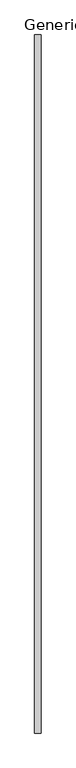
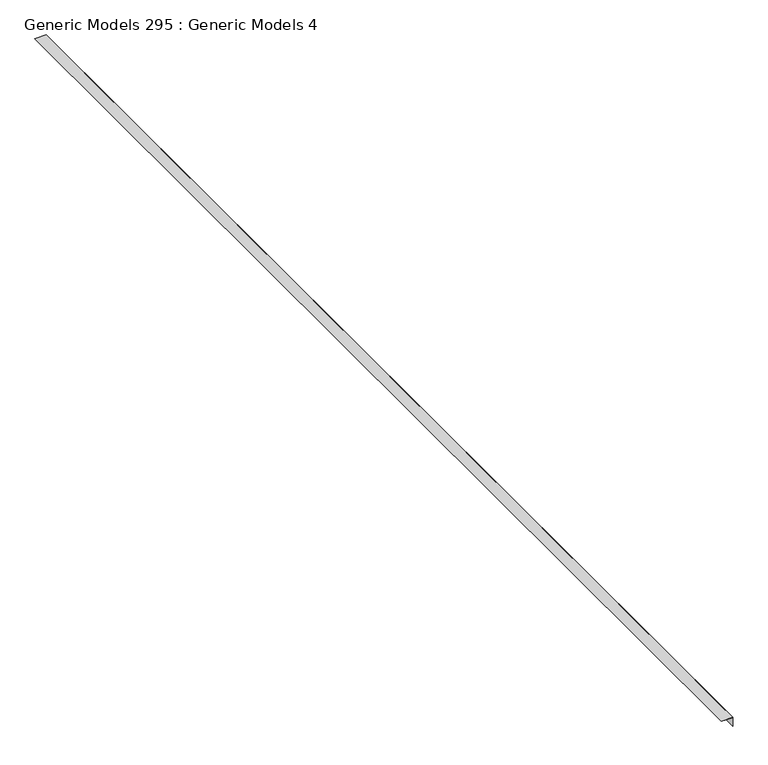
"""IFC4 building model written with IfcOpenShell, lengths in millimetres: proxy geometry, Generic Models 295 : Generic Models 4."""

from ifc_helpers import new_model, si_unit, frame, origin, place, context, project, spatial, polyline, outline, extrude, source, transform, mapped, element, save


def generic_models_295_generic_models_4_67822905(model_context):
    return source(origin(), model_context, "Body", "SweptSolid", [
        extrude(outline(polyline([(123327.4475314, 87413.1799276), (123245.6614247, 87413.1799276), (123245.6614247, 87413.9736776), (123328.2412814, 87413.9736776), (123328.2412814, 87313.815657), (123327.4475314, 87313.815657), (123327.4475314, 87413.1799276)])), frame((0.0, 16287.5029335, 0.0), z_axis=(0.0, 1.0, 0.0), x_axis=(0.0, 0.0, 1.0)), (0.0, 0.0, 1.0), 10638.2238531),
    ])


if __name__ == "__main__":
    model = new_model("IFC4")
    model_context = context("Model", 3, world=origin())
    ifc_project = project(units=[si_unit("LENGTHUNIT", "METRE", prefix="MILLI")], contexts=[model_context])
    site = spatial("IfcSite", under=ifc_project)
    building = spatial("IfcBuilding", under=site)
    placement = place(None, origin())
    generic_models_295_generic_models_4_shape = generic_models_295_generic_models_4_67822905(model_context)
    element("IfcBuildingElementProxy", 1, Name="Generic Models 295 : Generic Models 4", ObjectType="Generic Models 295 : Generic Models 4", at=placement, inside=building, context=model_context, shape_type="MappedRepresentation", body=[
        mapped(generic_models_295_generic_models_4_shape, transform((0.0, 0.0, 0.0), x_axis=(1.0, 0.0, 0.0), y_axis=(0.0, 1.0, 0.0), z_axis=(0.0, 0.0, 1.0))),
    ])
    save(model, "model.ifc")

# Revit data of these elements
# Element 1 (IfcBuildingElementProxy, "Generic Models 295 : Generic Models 4")
#   Materials on its faces: "_SELF ADHERED MEMBRANE W/ END DAMS WHERE POSSIBLE"
# Materials
#   "_SELF ADHERED MEMBRANE W/ END DAMS WHERE POSSIBLE": class "Generic", colour RGB 253 192 103, transparency 0, Cost = 0
